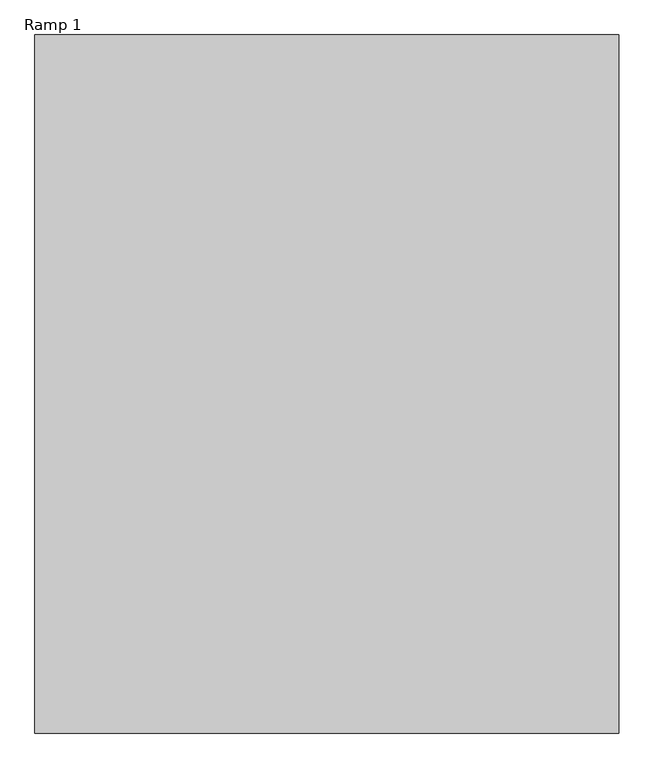
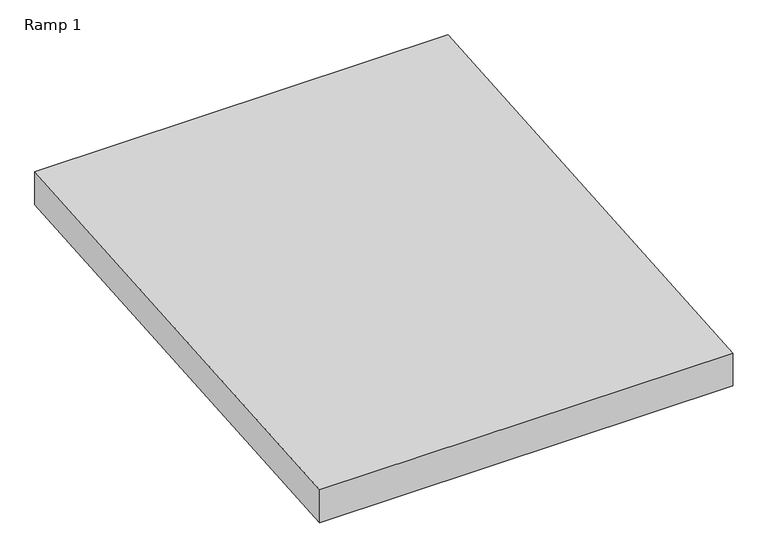
"""IFC4 building model written with IfcOpenShell, lengths in millimetres: ramp geometry, Ramp 1."""

from ifc_helpers import new_model, si_unit, frame, origin, place, context, project, spatial, polyline, outline, extrude, source, transform, mapped, element, save


def ramp_1_66d68c1d(model_context):
    return source(origin(), model_context, "Body", "SweptSolid", [
        extrude(outline(polyline([(-178.9025016, 40.0), (1960.7723822, 200.0), (1960.7723822, 49.5812066), (-178.9025016, -110.4187934), (-178.9025016, 40.0)])), frame((5764.7203549, 0.0, 0.0), z_axis=(1.0, 0.0, 0.0), x_axis=(0.0, 1.0, 0.0)), (0.0, 0.0, 1.0), 1790.0),
    ])


if __name__ == "__main__":
    model = new_model("IFC4")
    model_context = context("Model", 3, world=origin())
    ifc_project = project(units=[si_unit("LENGTHUNIT", "METRE", prefix="MILLI")], contexts=[model_context])
    site = spatial("IfcSite", under=ifc_project)
    building = spatial("IfcBuilding", under=site)
    placement = place(None, origin())
    ramp_1_shape = ramp_1_66d68c1d(model_context)
    element("IfcRamp", 1, ObjectType="Ramp 1", at=placement, inside=building, context=model_context, shape_type="MappedRepresentation", body=[
        mapped(ramp_1_shape, transform((0.0, 0.0, 0.0), x_axis=(1.0, 0.0, 0.0), y_axis=(0.0, 1.0, 0.0), z_axis=(0.0, 0.0, 1.0))),
    ])
    save(model, "model.ifc")
